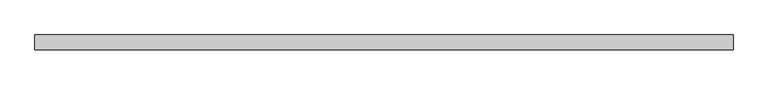
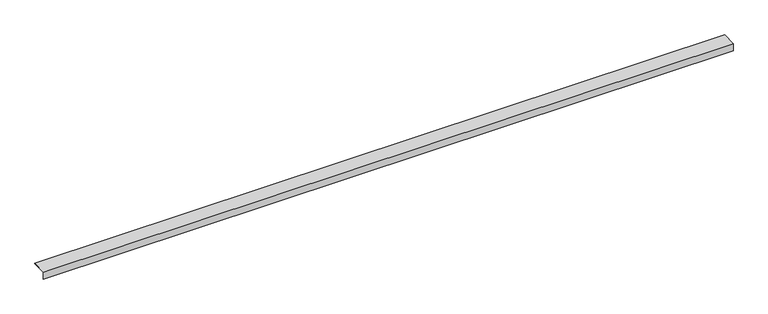
"""IFC4 building model written with IfcOpenShell, lengths in millimetres: proxy geometry, Generic Models 7:Generic Models 1:8:Generic Models 1:8 : Generic Models 7:Generic Models 1:337419:17 : Generic Models 7:Generic Models 1:8:Generic Models 1:8 : Generic Models 7:Generic Models 1:337419:315935."""

from ifc_helpers import new_model, si_unit, frame, origin, place, context, project, spatial, polyline, outline, extrude, source, transform, mapped, element, save


def generic_models_6e0294e0(model_context):
    return source(origin(), model_context, "Body", "SweptSolid", [
        extrude(outline(polyline([(-579120.6092291, 3665.1571615), (-579124.1195091, 3665.1571615), (-579124.1195091, 3715.9571615), (-579021.2760575, 3720.2423053), (-579021.1299226, 3716.7350684), (-579120.6092291, 3712.5900973), (-579120.6092291, 3665.1571615)])), frame((591306.0367239, 0.0, 0.0), z_axis=(1.0, 0.0, 0.0), x_axis=(0.0, 1.0, 0.0)), (0.0, 0.0, 1.0), 4876.8),
    ])


if __name__ == "__main__":
    model = new_model("IFC4")
    model_context = context("Model", 3, world=origin())
    ifc_project = project(units=[si_unit("LENGTHUNIT", "METRE", prefix="MILLI")], contexts=[model_context])
    site = spatial("IfcSite", under=ifc_project)
    building = spatial("IfcBuilding", under=site)
    placement = place(None, origin())
    generic_models_shape = generic_models_6e0294e0(model_context)
    element("IfcBuildingElementProxy", 1, Name="Generic Models 7:Generic Models 1:8:Generic Models 1:8 : Generic Models 7:Generic Models 1:337419:17 : Generic Models 7:Generic Models 1:8:Generic Models 1:8 : Generic Models 7:Generic Models 1:337419:315935", ObjectType="Generic Models 7:Generic Models 1:8:Generic Models 1:8 : Generic Models 7:Generic Models 1:337419:17 : Generic Models 7:Generic Models 1:8:Generic Models 1:8 : Generic Models 7:Generic Models 1:337419:315935", at=placement, inside=building, context=model_context, shape_type="MappedRepresentation", body=[
        mapped(generic_models_shape, transform((0.0, 0.0, 0.0), x_axis=(1.0, 0.0, 0.0), y_axis=(0.0, 1.0, 0.0), z_axis=(0.0, 0.0, 1.0))),
    ])
    save(model, "model.ifc")

# Revit data of these elements
# Type "Generic Models 7:Generic Models 1:8:Generic Models 1:8 : Generic Models 7:Generic Models 1:337419:17 : Generic Models 7:Generic Models 1:8:Generic Models 1:8 : Generic Models 7:Generic Models 1:337419:315935"
#   NameOverride = "Generic Models 7:Generic Models 1:8:Generic Models 1:8 : Generic Models 7:Generic Models 1:337419:315935"
#   ObjectTypeOverride = "Generic Models 1:8 : Generic Models 7:Generic Models 1:337419"
#   Reference = "Generic Models 1"
#   Tag = "315935"
# Element 1 (IfcBuildingElementProxy, "Generic Models 7:Generic Models 1:8:Generic Models 1:8 : Generic Models 7:Generic Models 1:337419:17 : Generic Models 7:Generic Models 1:8:Generic Models 1:8 : Generic Models 7:Generic Models 1:337419:315935")
#   Materials on its faces: "11 GA. ALUM. BRAKE METAL (ALIGN WITH B.M. @ STOREFRONT/RESIN/POLYCARBONATE)"
# Materials
#   "11 GA. ALUM. BRAKE METAL (ALIGN WITH B.M. @ STOREFRONT/RESIN/POLYCARBONATE)": class "Unassigned", colour RGB 210 209 208, transparency 0, Cost = 0
